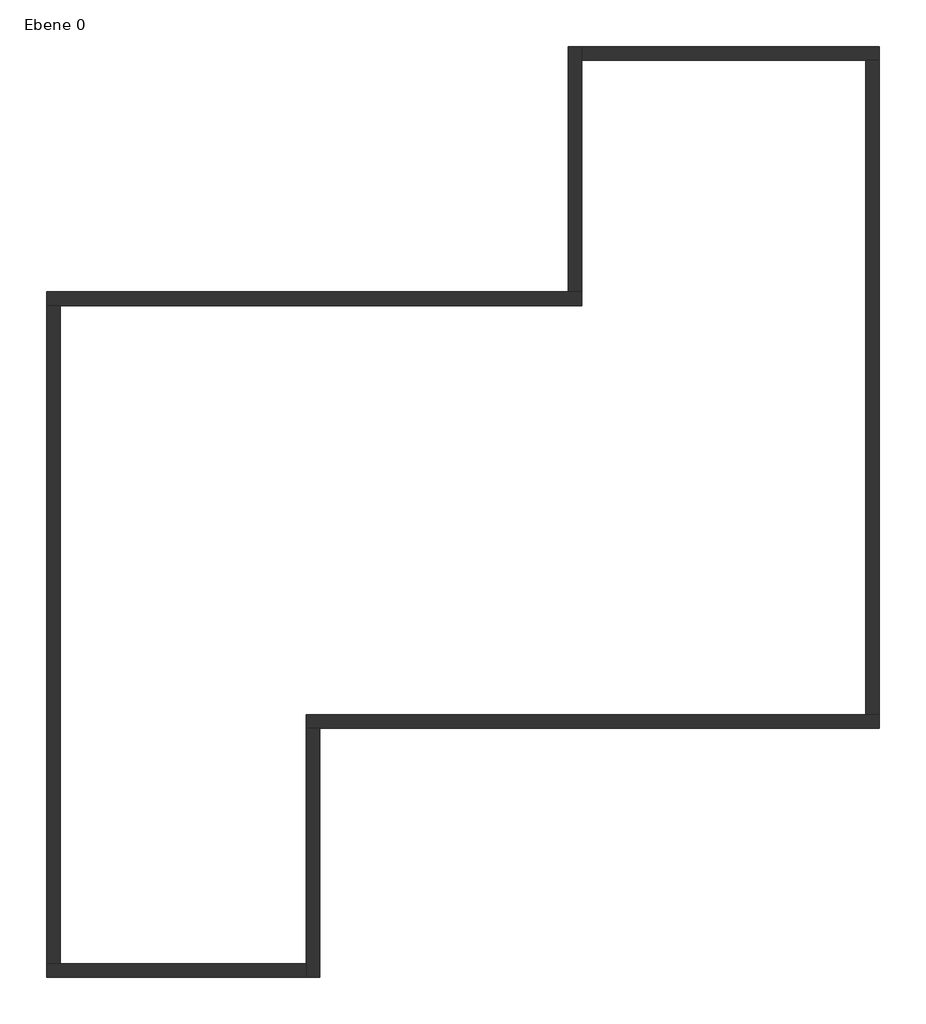
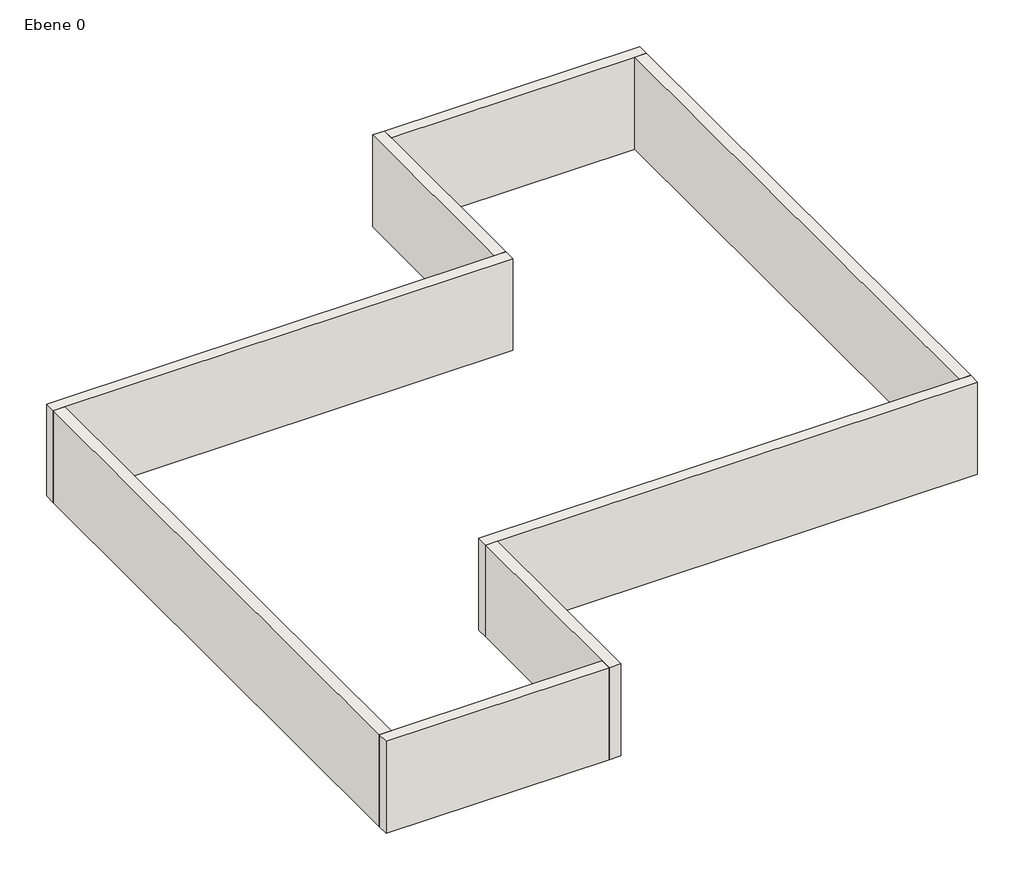
# One storey: 8 walls.
"""IFC4 building model written with IfcOpenShell, lengths in millimetres."""

import ifcopenshell
import ifcopenshell.guid

model = None  # the IFC model being written
_history = None  # IfcOwnerHistory: only IFC2X3 demands one
_inside = {}  # id of a spatial element -> (the spatial element, [elements in it])
_under = {}  # id of a project, library or spatial element -> (it, [spatial elements below it])
_declared = {}  # id of a project -> (the project, [libraries it declares])
_typed = {}  # id of a type object -> (the type object, [elements of that type])
_made_of = {}  # id of a material, layer set ... -> (it, [elements and type objects made of it])


def new_model(schema):
    """Start an empty IFC model of exactly this schema.

    Asked for "IFC4X3", IfcOpenShell would pick the latest addendum, in which some entities
    have other attributes; the version numbers below select the first issue.
    IFC2X3 requires an IfcOwnerHistory on every rooted entity: one is made here for all.
    """
    global model, _history
    if schema == "IFC4X3":
        model = ifcopenshell.file(schema_version=(4, 3, 0, 0))
    else:
        model = ifcopenshell.file(schema=schema)
    _inside.clear()
    _under.clear()
    _declared.clear()
    _typed.clear()
    _made_of.clear()
    _history = None
    if model.schema == "IFC2X3":
        org = make("IfcOrganization", Name="unknown")
        user = make(
            "IfcPersonAndOrganization",
            ThePerson=make("IfcPerson", FamilyName="unknown"),
            TheOrganization=org,
        )
        app = make(
            "IfcApplication",
            ApplicationDeveloper=org,
            Version="unknown",
            ApplicationFullName="unknown",
            ApplicationIdentifier="unknown",
        )
        _history = make(
            "IfcOwnerHistory",
            OwningUser=user,
            OwningApplication=app,
            ChangeAction="ADDED",
            CreationDate=0,
        )
    return model


def make(cls, **values):
    """One entity of the class cls with the attributes given. An attribute that is None is left unset."""
    return model.create_entity(
        cls, **{name: value for name, value in values.items() if value is not None}
    )


def rooted(cls, **values):
    """An entity with a GlobalId (a new one), such as an element, a storey or a relation."""
    return make(cls, GlobalId=ifcopenshell.guid.new(), OwnerHistory=_history, **values)


def si_unit(unit_type, name, prefix=None):
    """IfcSIUnit, for example si_unit("LENGTHUNIT", "METRE", prefix="MILLI")."""
    return make("IfcSIUnit", UnitType=unit_type, Prefix=prefix, Name=name)


def assignment(units):
    """IfcUnitAssignment: the units of a project."""
    return None if units is None else make("IfcUnitAssignment", Units=units)


def point(xyz):
    """IfcCartesianPoint."""
    return None if xyz is None else make("IfcCartesianPoint", Coordinates=xyz)


def direction(xyz):
    """IfcDirection."""
    return None if xyz is None else make("IfcDirection", DirectionRatios=xyz)


def frame(location, z_axis=None, x_axis=None):
    """IfcAxis2Placement3D, a coordinate frame: its origin and axes. An axis left out is left unset."""
    return make(
        "IfcAxis2Placement3D",
        Location=point(location),
        Axis=direction(z_axis),
        RefDirection=direction(x_axis),
    )


def origin():
    """The frame at (0, 0, 0) with its axes left unset."""
    return frame((0.0, 0.0, 0.0))


def origin_with_axes():
    """The frame at (0, 0, 0) with the z axis (0, 0, 1) and the x axis (1, 0, 0) written out."""
    return frame((0.0, 0.0, 0.0), z_axis=(0.0, 0.0, 1.0), x_axis=(1.0, 0.0, 0.0))


def place(relative_to, where):
    """IfcLocalPlacement: puts the frame where relative to a parent placement (None: the world)."""
    return make(
        "IfcLocalPlacement", PlacementRelTo=relative_to, RelativePlacement=where
    )


def context(
    kind, dimensions, precision=None, world=None, true_north=None, identifier=None
):
    """IfcGeometricRepresentationContext, for example the 3D "Model" context."""
    return make(
        "IfcGeometricRepresentationContext",
        ContextIdentifier=identifier,
        ContextType=kind,
        CoordinateSpaceDimension=dimensions,
        Precision=precision,
        WorldCoordinateSystem=world,
        TrueNorth=true_north,
    )


def project(units=None, contexts=None):
    """IfcProject with its units and contexts."""
    return rooted(
        "IfcProject",
        Name="project",
        RepresentationContexts=contexts,
        UnitsInContext=assignment(units),
    )


def spatial(cls, under=None, at=None, **own):
    """A site, building, storey or space (cls), placed at a placement, below another one or the project."""
    s = rooted(cls, ObjectPlacement=at, **own)
    if under is not None:
        _under.setdefault(under.id(), (under, []))[1].append(s)
    return s


def polyline(points):
    """IfcPolyline through the points."""
    return make("IfcPolyline", Points=[point(p) for p in points])


def outline(outer, holes=None, kind="AREA"):
    """IfcArbitraryClosedProfileDef: a profile drawn as a closed curve; with holes, ...WithVoids."""
    if holes is None:
        return make("IfcArbitraryClosedProfileDef", ProfileType=kind, OuterCurve=outer)
    return make(
        "IfcArbitraryProfileDefWithVoids",
        ProfileType=kind,
        OuterCurve=outer,
        InnerCurves=holes,
    )


def extrude(swept, where, along, depth):
    """IfcExtrudedAreaSolid: the profile swept, set in the frame where, extruded along a direction by depth."""
    return make(
        "IfcExtrudedAreaSolid",
        SweptArea=swept,
        Position=where,
        ExtrudedDirection=direction(along),
        Depth=depth,
    )


def faces_of(points, faces, orient=None, outer=None):
    """IfcFace entities. A face is a list of loops; a loop is a list of indices into points, from 0.

    orient and outer hold one flag for each loop. By default every Orientation is true, the
    first loop of a face is its IfcFaceOuterBound and the others are IfcFaceBound.
    """
    made = []
    for i, loops in enumerate(faces):
        bounds = []
        for j, loop in enumerate(loops):
            is_outer = j == 0 if outer is None else outer[i][j]
            bounds.append(
                make(
                    "IfcFaceOuterBound" if is_outer else "IfcFaceBound",
                    Bound=make("IfcPolyLoop", Polygon=[points[k] for k in loop]),
                    Orientation=True if orient is None else orient[i][j],
                )
            )
        made.append(make("IfcFace", Bounds=bounds))
    return made


def faceted_brep(points, faces, orient=None, outer=None, voids=None):
    """IfcFacetedBrep: a solid bounded by flat faces; with voids (closed shells), ...WithVoids."""
    shared = [point(p) for p in points]
    hull = make("IfcClosedShell", CfsFaces=faces_of(shared, faces, orient, outer))
    if voids is None:
        return make("IfcFacetedBrep", Outer=hull)
    return make(
        "IfcFacetedBrepWithVoids",
        Outer=hull,
        Voids=[
            make(cls, CfsFaces=faces_of(shared, fs, o, b)) for cls, fs, o, b in voids
        ],
    )


def shape(context_of_items, identifier, shape_type, items):
    """IfcShapeRepresentation: the items that make up one representation, for example the "Body"."""
    return make(
        "IfcShapeRepresentation",
        ContextOfItems=context_of_items,
        RepresentationIdentifier=identifier,
        RepresentationType=shape_type,
        Items=items,
    )


def made_of(thing, what):
    """Note that an element or type object is made of a material, layer set ...; save() writes the relation."""
    if what is not None:
        _made_of.setdefault(what.id(), (what, []))[1].append(thing)
    return thing


def element(
    cls,
    number,
    at=None,
    inside=None,
    cuts=None,
    type_object=None,
    material=None,
    context=None,
    identifier="Body",
    shape_type=None,
    held_by="IfcProductDefinitionShape",
    body=None,
    shapes=None,
    **own,
):
    """One element of the class cls, such as IfcWall. Its Tag is "e" and its number.

    at: its placement. inside: the storey or other place that contains it. cuts: it is an
    opening in that element (IfcRelVoidsElement). A single representation is given by context,
    identifier, shape_type and body (its items); several are given by shapes. held_by: the class
    of the entity that holds the representations. save() writes the other relations.
    """
    e = rooted(cls, Tag="e%d" % number, ObjectPlacement=at, **own)
    if body is not None:
        shapes = [shape(context, identifier, shape_type, body)]
    if shapes is not None:
        e.Representation = make(held_by, Representations=shapes)
    if inside is not None:
        _inside.setdefault(inside.id(), (inside, []))[1].append(e)
    if cuts is not None:
        rooted(
            "IfcRelVoidsElement", RelatingBuildingElement=cuts, RelatedOpeningElement=e
        )
    if type_object is not None:
        _typed.setdefault(type_object.id(), (type_object, []))[1].append(e)
    return made_of(e, material)


def aggregate(whole, parts):
    """IfcRelAggregates: a whole, such as a stair, and the parts it consists of."""
    return rooted("IfcRelAggregates", RelatingObject=whole, RelatedObjects=parts)


def save(model, path):
    """Write the relations noted so far, then the file.

    IfcRelAggregates (storeys below a building ...), IfcRelContainedInSpatialStructure (elements
    in a storey), IfcRelDefinesByType, IfcRelAssociatesMaterial and IfcRelDeclares: one each for
    every whole, place, type object, material and project.
    """
    for whole, parts in _under.values():
        aggregate(whole, parts)
    for where, things in _inside.values():
        rooted(
            "IfcRelContainedInSpatialStructure",
            RelatedElements=things,
            RelatingStructure=where,
        )
    for kind, things in _typed.values():
        rooted("IfcRelDefinesByType", RelatedObjects=things, RelatingType=kind)
    for what, things in _made_of.values():
        rooted("IfcRelAssociatesMaterial", RelatedObjects=things, RelatingMaterial=what)
    for by, libraries in _declared.values():
        rooted("IfcRelDeclares", RelatingContext=by, RelatedDefinitions=libraries)
    model.write(path)


model = new_model("IFC4")

# Units and contexts
model_context = context("Model", 3, world=origin())
ifc_project = project(units=[si_unit("LENGTHUNIT", "METRE", prefix="MILLI")], contexts=[model_context])

# Site, building, storey
site = spatial("IfcSite", under=ifc_project)
building = spatial("IfcBuilding", under=site)
storey = spatial("IfcBuildingStorey", under=building, Name="Ebene 0", Elevation=0.0)

# Walls
placement = place(None, origin())
element("IfcWall", 1, ObjectType="MW 24.0 WD 12.0", at=placement, inside=storey, context=model_context, shape_type="Brep", body=[
    faceted_brep([(-13369.6797169, 6985.6067473, 0.0), (-13009.6797169, 6985.6067473, 0.0), (810.3202831, 6985.6067473, 0.0), (810.3202831, 6985.6067473, 3000.0), (-13009.6797169, 6985.6067473, 3000.0), (-13369.6797169, 6985.6067473, 3000.0), (-13369.6797169, 7345.6067473, 0.0), (-13369.6797169, 7345.6067473, 3000.0), (450.3202831, 7345.6067473, 3000.0), (810.3202831, 7345.6067473, 3000.0), (810.3202831, 7345.6067473, 0.0), (450.3202831, 7345.6067473, 0.0)], [[[0, 1, 2, 3, 4, 5]], [[6, 7, 8, 9, 10, 11]], [[2, 1, 0, 6, 11, 10]], [[5, 4, 3, 9, 8, 7]], [[0, 5, 7, 6]], [[3, 2, 10, 9]]]),
])
element("IfcWall", 2, ObjectType="MW 24.0 WD 12.0", at=placement, inside=storey, context=model_context, shape_type="SweptSolid", body=[
    extrude(outline(polyline([(-13009.6797169, 6985.6067473), (-13009.6797169, -10454.3932527), (-13369.6797169, -10454.3932527), (-13369.6797169, 6985.6067473), (-13009.6797169, 6985.6067473)])), origin_with_axes(), (0.0, 0.0, 1.0), 3000.0),
])
element("IfcWall", 3, ObjectType="MW 24.0 WD 12.0", at=placement, inside=storey, context=model_context, shape_type="Brep", body=[
    faceted_brep([(8690.3202831, -3854.3932527, 0.0), (8330.3202831, -3854.3932527, 0.0), (-6489.6797169, -3854.3932527, 0.0), (-6489.6797169, -3854.3932527, 3000.0), (8330.3202831, -3854.3932527, 3000.0), (8690.3202831, -3854.3932527, 3000.0), (8690.3202831, -4214.3932527, 0.0), (8690.3202831, -4214.3932527, 3000.0), (-6129.6797169, -4214.3932527, 3000.0), (-6489.6797169, -4214.3932527, 3000.0), (-6489.6797169, -4214.3932527, 0.0), (-6129.6797169, -4214.3932527, 0.0)], [[[0, 1, 2, 3, 4, 5]], [[6, 7, 8, 9, 10, 11]], [[2, 1, 0, 6, 11, 10]], [[5, 4, 3, 9, 8, 7]], [[0, 5, 7, 6]], [[3, 2, 10, 9]]]),
])
element("IfcWall", 4, ObjectType="MW 24.0 WD 12.0", at=placement, inside=storey, context=model_context, shape_type="SweptSolid", body=[
    extrude(outline(polyline([(8330.3202831, -3854.3932527), (8330.3202831, 13485.6067473), (8690.3202831, 13485.6067473), (8690.3202831, -3854.3932527), (8330.3202831, -3854.3932527)])), origin_with_axes(), (0.0, 0.0, 1.0), 3000.0),
])
element("IfcWall", 5, ObjectType="MW 24.0 WD 12.0", at=placement, inside=storey, context=model_context, shape_type="Brep", body=[
    faceted_brep([(810.3202831, 7345.6067473, 0.0), (810.3202831, 13485.6067473, 0.0), (810.3202831, 13845.6067473, 0.0), (810.3202831, 13845.6067473, 3000.0), (810.3202831, 13485.6067473, 3000.0), (810.3202831, 7345.6067473, 3000.0), (450.3202831, 7345.6067473, 0.0), (450.3202831, 7345.6067473, 3000.0), (450.3202831, 13845.6067473, 3000.0), (450.3202831, 13845.6067473, 0.0)], [[[0, 1, 2, 3, 4, 5]], [[6, 7, 8, 9]], [[2, 1, 0, 6, 9]], [[5, 4, 3, 8, 7]], [[3, 2, 9, 8]], [[0, 5, 7, 6]]]),
])
element("IfcWall", 6, ObjectType="MW 24.0 WD 12.0", at=placement, inside=storey, context=model_context, shape_type="Brep", body=[
    faceted_brep([(810.3202831, 13485.6067473, 0.0), (8330.3202831, 13485.6067473, 0.0), (8690.3202831, 13485.6067473, 0.0), (8690.3202831, 13485.6067473, 3000.0), (8330.3202831, 13485.6067473, 3000.0), (810.3202831, 13485.6067473, 3000.0), (810.3202831, 13845.6067473, 0.0), (810.3202831, 13845.6067473, 3000.0), (8690.3202831, 13845.6067473, 3000.0), (8690.3202831, 13845.6067473, 0.0)], [[[0, 1, 2, 3, 4, 5]], [[6, 7, 8, 9]], [[2, 1, 0, 6, 9]], [[5, 4, 3, 8, 7]], [[0, 5, 7, 6]], [[3, 2, 9, 8]]]),
])
element("IfcWall", 7, ObjectType="MW 24.0 WD 12.0", at=placement, inside=storey, context=model_context, shape_type="Brep", body=[
    faceted_brep([(-6489.6797169, -4214.3932527, 0.0), (-6489.6797169, -10454.3932527, 0.0), (-6489.6797169, -10814.3932527, 0.0), (-6489.6797169, -10814.3932527, 3000.0), (-6489.6797169, -10454.3932527, 3000.0), (-6489.6797169, -4214.3932527, 3000.0), (-6129.6797169, -4214.3932527, 0.0), (-6129.6797169, -4214.3932527, 3000.0), (-6129.6797169, -10814.3932527, 3000.0), (-6129.6797169, -10814.3932527, 0.0)], [[[0, 1, 2, 3, 4, 5]], [[6, 7, 8, 9]], [[2, 1, 0, 6, 9]], [[5, 4, 3, 8, 7]], [[3, 2, 9, 8]], [[0, 5, 7, 6]]]),
])
element("IfcWall", 8, ObjectType="MW 24.0 WD 12.0", at=placement, inside=storey, context=model_context, shape_type="Brep", body=[
    faceted_brep([(-6489.6797169, -10454.3932527, 0.0), (-13009.6797169, -10454.3932527, 0.0), (-13369.6797169, -10454.3932527, 0.0), (-13369.6797169, -10454.3932527, 3000.0), (-13009.6797169, -10454.3932527, 3000.0), (-6489.6797169, -10454.3932527, 3000.0), (-6489.6797169, -10814.3932527, 0.0), (-6489.6797169, -10814.3932527, 3000.0), (-13369.6797169, -10814.3932527, 3000.0), (-13369.6797169, -10814.3932527, 0.0)], [[[0, 1, 2, 3, 4, 5]], [[6, 7, 8, 9]], [[2, 1, 0, 6, 9]], [[5, 4, 3, 8, 7]], [[0, 5, 7, 6]], [[3, 2, 9, 8]]]),
])

save(model, "model.ifc")

# Revit data of these elements
# Project information
#   Projektausgabedatum = "Projekt Datum"
#   Projektstatus = "Projektstatus"
#   Kundenname = "Bauherr"
#   Projektadresse = "Projektadresse"
#   Projektname = "Projektname"
#   Projektnummer = "Projektnummer"
#   Verfasser Firma 1 = "Firma 1"
#   Verfasser Firma 2 = "Firma 2"
#   Verfasser PLZ Ort = "PLZ Ort"
#   Verfasser Strasse = "Strasse"
#   Verfasser Telefon = "Telefon"
#   Verfasser Telefax = "Telefax"
#   Verfasser eMail = "E-Mail"
# Type "MW 24.0 WD 12.0"
#   Type Comments = "Mehrschaliges Mauerwerk"
#   Description = "Mauerwerk 24.0 cm, Wärmedämmung 12.0 cm"
#   Width = 0.360 m
#   Layers, outside or top first: 0.120 m "Wärmedämmung - Hart" (function 3); 0.240 m "Mauerwerk - Ziegel, verputzt" (function 1)
# Elements 1, 3 (IfcWall, "MW 24.0 WD 12.0")
#   Top Offset = 0.000 m
#   Base Offset = 0.000 m
#   wall height = 3.000 m
#   Phase Created = Phase 1
#   Base Constraint = Ebene 0
#   Top Constraint = Ebene 1
#   Materials on its faces: "Mauerwerk - Ziegel, verputzt", "Wärmedämmung - Hart", "Standard - Wand"
# Elements 2, 4 (IfcWall, "MW 24.0 WD 12.0")
#   Top Offset = 0.000 m
#   Base Offset = 0.000 m
#   wall height = 3.000 m
#   Phase Created = Phase 1
#   Base Constraint = Ebene 0
#   Top Constraint = Ebene 1
#   Materials on its faces: "Standard - Wand", "Mauerwerk - Ziegel, verputzt", "Wärmedämmung - Hart"
# Elements 5, 6, 7, 8 (IfcWall, "MW 24.0 WD 12.0")
#   Top Offset = 0.000 m
#   Base Offset = 0.000 m
#   wall height = 3.000 m
#   Phase Created = Phase 1
#   Base Constraint = Ebene 0
#   Top Constraint = Ebene 1
#   Materials on its faces: "Standard - Wand", "Wärmedämmung - Hart", "Mauerwerk - Ziegel, verputzt"
# Materials
#   "Wärmedämmung - Hart": class "Putz", colour RGB 255 255 255, transparency 0, Description = "Äußere Oberfläche"
#   "Mauerwerk - Ziegel, verputzt": class "Putz", colour RGB 247 247 247, transparency 0, Cost = 0
#   "Standard - Wand": class "Putz", colour RGB 128 128 128, transparency 0, Description = "Äußere Oberfläche"
